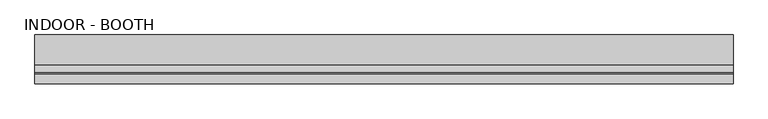
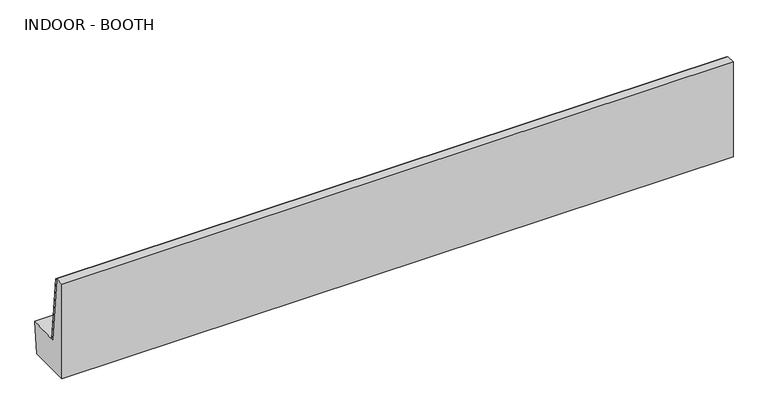
"""IFC4 building model written with IfcOpenShell, lengths in millimetres: furniture geometry, OD_CW_Booth : INDOOR - BOOTH."""

from ifc_helpers import new_model, si_unit, frame, origin, place, context, project, spatial, polyline, outline, extrude, source, transform, mapped, element, save


def indoor_booth_a2b8d8e1(model_context):
    return source(origin(), model_context, "Body", "SweptSolid", [
        extrude(outline(polyline([(0.0, -9357.0837874), (0.0, 0.0), (25.4, 0.0), (25.4, -9357.0837874), (0.0, -9357.0837874)])), frame((9375.8214923, -358.2049359, 438.8309433), z_axis=(0.0, -0.10452846326765197, 0.9945218953682735), x_axis=(0.0, -0.9945218953682735, -0.10452846326765197)), (0.0, 0.0, 1.0), 944.7333479),
        extrude(outline(polyline([(-609.6, 1397.0), (-484.4524721, 1397.0), (-382.9385128, 431.1591941), (43.0849153, 453.4861359), (3.4100193, 0.0), (-609.6, 0.0), (-609.6, 1397.0)])), frame((18.7377049, 0.0, 0.0), z_axis=(1.0, 0.0, 0.0), x_axis=(0.0, 1.0, 0.0)), (0.0, 0.0, 1.0), 9357.0837874),
    ])


if __name__ == "__main__":
    model = new_model("IFC4")
    model_context = context("Model", 3, world=origin())
    ifc_project = project(units=[si_unit("LENGTHUNIT", "METRE", prefix="MILLI")], contexts=[model_context])
    site = spatial("IfcSite", under=ifc_project)
    building = spatial("IfcBuilding", under=site)
    placement = place(None, origin())
    indoor_booth_shape = indoor_booth_a2b8d8e1(model_context)
    element("IfcFurniture", 1, ObjectType="OD_CW_Booth : INDOOR - BOOTH", at=placement, inside=building, context=model_context, shape_type="MappedRepresentation", body=[
        mapped(indoor_booth_shape, transform((0.0, 0.0, 0.0), x_axis=(1.0, 0.0, 0.0), y_axis=(0.0, 1.0, 0.0), z_axis=(0.0, 0.0, 1.0))),
    ])
    save(model, "model.ifc")

# Revit data of these elements
# Type "OD_CW_Booth : INDOOR - BOOTH"
#   Type Mark = "TYPE - INDOOR - BOOTH"
#   Width = 4' - 0"
#   OD_CW_Width [instance default] = 2' - 10"
#   OD_CW_Length [instance default] = 26' - 1 83/256"
#   OD_CW_Height [instance default] = 2' - 3"
#   Height = 3' - 0"
#   Depth = 2' - 0"
#   Seating Count [instance default] = 10
#   Seating Count [instance default] = 10
#   back = WOOD VENEER
#   OD_CW_Material_Front Panel [instance default] = none
#   OD_CW_Material_Body [instance default] = none
# Element 1 (IfcFurniture, "OD_CW_Booth : INDOOR - BOOTH")
#   OD_CW_Length = 30' - 8.38913"
#   Seating Count = 11
#   OD_CW_Material_Body = WOOD-OAKFIRE
#   Materials on its faces: "WOOD-OAKFIRE", "WOOD VENEER"
# Materials
#   "WOOD VENEER": class "Miscellaneous", colour RGB 164 164 164, transparency 0, Cost = 0
#   "WOOD-OAKFIRE": class "Wood", colour RGB 198 202 183, transparency 0, Description = "Generic wood", Cost = 0
